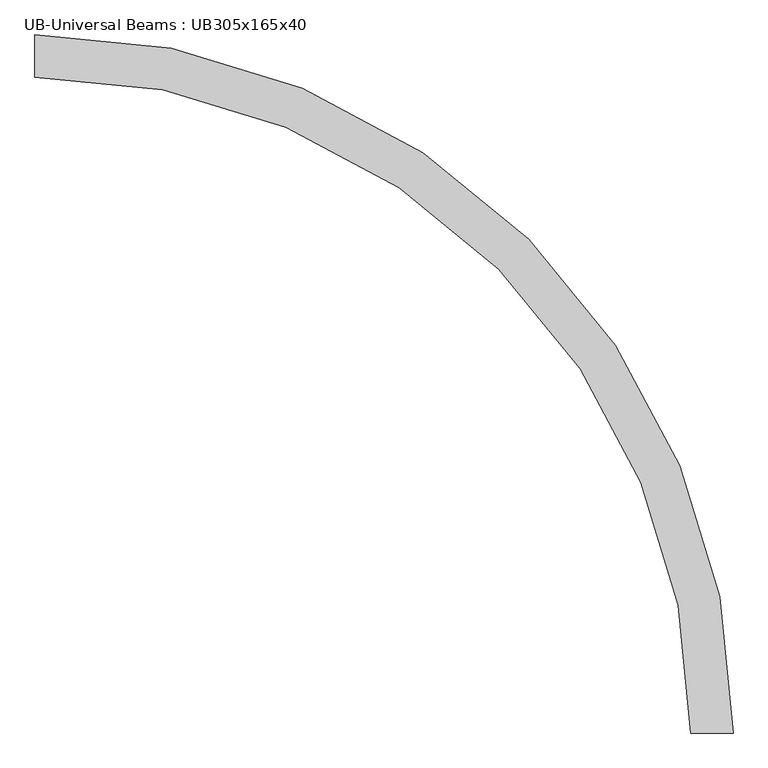
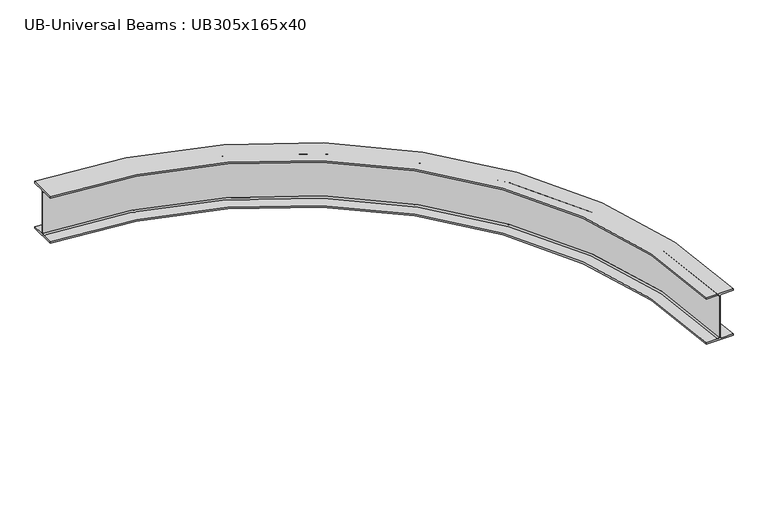
"""IFC4 building model written with IfcOpenShell, lengths in millimetres: beam geometry, UB-Universal Beams : UB305x165x40."""

from ifc_helpers import new_model, si_unit, point, frame, origin, place, context, project, spatial, polyline, circle_curve, ellipse_curve, trimmed, source, transform, mapped, element, save
from ifc_brep_helpers import plane_surface, cylinder_surface, revolved_surface, advanced_brep


def ub_universal_beams_ub305x165x40_a7bc032b(model_context):
    return source(origin(), model_context, "Body", "AdvancedBrep", [
        advanced_brep(
        [(2724.4689627, -2641.9689627, -141.5), (2653.8689627, -2641.9689627, -141.5), (2644.9689627, -2641.9689627, -132.6), (2644.9689627, -2641.9689627, 132.6), (2653.8689627, -2641.9689627, 141.5), (2724.4689627, -2641.9689627, 141.5), (2724.4689627, -2641.9689627, 151.7), (2559.4689627, -2641.9689627, 151.7), (2559.4689627, -2641.9689627, 141.5), (2630.0689627, -2641.9689627, 141.5), (2638.9689627, -2641.9689627, 132.6), (2638.9689627, -2641.9689627, -132.6), (2630.0689627, -2641.9689627, -141.5), (2559.4689627, -2641.9689627, -141.5), (2559.4689627, -2641.9689627, -151.7), (2724.4689627, -2641.9689627, -151.7), (0.0, 82.5, -141.5), (0.0, 82.5, -151.7), (0.0, -82.5, -151.7), (0.0, -82.5, -141.5), (0.0, -11.9, -141.5), (0.0, -3.0, -132.6), (0.0, -3.0, 132.6), (0.0, -11.9, 141.5), (0.0, -82.5, 141.5), (0.0, -82.5, 151.7), (0.0, 82.5, 151.7), (0.0, 82.5, 141.5), (0.0, 11.9, 141.5), (0.0, 3.0, 132.6), (0.0, 3.0, -132.6), (0.0, 11.9, -141.5)],
        [
            (0, 1),
            (1, 2, circle_curve(frame((2653.8689627, -2641.9689627, -132.6), z_axis=(0.0, 1.0, 0.0), x_axis=(-1.0, 0.0, 0.0)), 8.9)),
            (2, 3),
            (3, 4, circle_curve(frame((2653.8689627, -2641.9689627, 132.6), z_axis=(0.0, 1.0, 0.0), x_axis=(-1.0, 0.0, 0.0)), 8.9)),
            (4, 5),
            (5, 6),
            (6, 7),
            (7, 8),
            (8, 9),
            (9, 10, circle_curve(frame((2630.0689627, -2641.9689627, 132.6), z_axis=(0.0, 1.0, 0.0), x_axis=(-1.0, 0.0, 0.0)), 8.9)),
            (10, 11),
            (11, 12, circle_curve(frame((2630.0689627, -2641.9689627, -132.6), z_axis=(0.0, 1.0, 0.0), x_axis=(-1.0, 0.0, 0.0)), 8.9)),
            (12, 13),
            (13, 14),
            (14, 15),
            (15, 0),
            (16, 17),
            (17, 18),
            (18, 19),
            (19, 20),
            (20, 21, circle_curve(frame((0.0, -11.9, -132.6), z_axis=(1.0, 0.0, 0.0), x_axis=(0.0, -1.0, 0.0)), 8.9)),
            (21, 22),
            (22, 23, circle_curve(frame((0.0, -11.9, 132.6), z_axis=(1.0, 0.0, 0.0), x_axis=(0.0, -1.0, 0.0)), 8.9)),
            (23, 24),
            (24, 25),
            (25, 26),
            (26, 27),
            (27, 28),
            (28, 29, circle_curve(frame((0.0, 11.9, 132.6), z_axis=(1.0, 0.0, 0.0), x_axis=(0.0, -1.0, 0.0)), 8.9)),
            (29, 30),
            (30, 31, circle_curve(frame((0.0, 11.9, -132.6), z_axis=(1.0, 0.0, 0.0), x_axis=(0.0, -1.0, 0.0)), 8.9)),
            (31, 16),
            (0, 16, circle_curve(frame((0.0, -2641.9689627, -141.5), z_axis=(0.0, 0.0, 1.0), x_axis=(0.0, 1.0, 0.0)), 2724.4689627)),
            (31, 1, circle_curve(frame((0.0, -2641.9689627, -141.5), z_axis=(0.0, 0.0, -1.0), x_axis=(0.0, 1.0, 0.0)), 2653.8689627)),
            (30, 2, circle_curve(frame((0.0, -2641.9689627, -132.6), z_axis=(0.0, 0.0, -1.0), x_axis=(0.0, 1.0, 0.0)), 2644.9689627)),
            (29, 3, circle_curve(frame((0.0, -2641.9689627, 132.6), z_axis=(0.0, 0.0, -1.0), x_axis=(0.0, 1.0, 0.0)), 2644.9689627)),
            (28, 4, circle_curve(frame((0.0, -2641.9689627, 141.5), z_axis=(0.0, 0.0, -1.0), x_axis=(0.0, 1.0, 0.0)), 2653.8689627)),
            (27, 5, circle_curve(frame((0.0, -2641.9689627, 141.5), z_axis=(0.0, 0.0, -1.0), x_axis=(0.0, 1.0, 0.0)), 2724.4689627)),
            (26, 6, circle_curve(frame((0.0, -2641.9689627, 151.7), z_axis=(0.0, 0.0, -1.0), x_axis=(0.0, 1.0, 0.0)), 2724.4689627)),
            (25, 7, circle_curve(frame((0.0, -2641.9689627, 151.7), z_axis=(0.0, 0.0, -1.0), x_axis=(0.0, 1.0, 0.0)), 2559.4689627)),
            (24, 8, circle_curve(frame((0.0, -2641.9689627, 141.5), z_axis=(0.0, 0.0, -1.0), x_axis=(0.0, 1.0, 0.0)), 2559.4689627)),
            (23, 9, circle_curve(frame((0.0, -2641.9689627, 141.5), z_axis=(0.0, 0.0, -1.0), x_axis=(0.0, 1.0, 0.0)), 2630.0689627)),
            (22, 10, circle_curve(frame((0.0, -2641.9689627, 132.6), z_axis=(0.0, 0.0, -1.0), x_axis=(0.0, 1.0, 0.0)), 2638.9689627)),
            (21, 11, circle_curve(frame((0.0, -2641.9689627, -132.6), z_axis=(0.0, 0.0, -1.0), x_axis=(0.0, 1.0, 0.0)), 2638.9689627)),
            (20, 12, circle_curve(frame((0.0, -2641.9689627, -141.5), z_axis=(0.0, 0.0, -1.0), x_axis=(0.0, 1.0, 0.0)), 2630.0689627)),
            (19, 13, circle_curve(frame((0.0, -2641.9689627, -141.5), z_axis=(0.0, 0.0, -1.0), x_axis=(0.0, 1.0, 0.0)), 2559.4689627)),
            (18, 14, circle_curve(frame((0.0, -2641.9689627, -151.7), z_axis=(0.0, 0.0, -1.0), x_axis=(0.0, 1.0, 0.0)), 2559.4689627)),
            (17, 15, circle_curve(frame((0.0, -2641.9689627, -151.7), z_axis=(0.0, 0.0, -1.0), x_axis=(0.0, 1.0, 0.0)), 2724.4689627)),
        ],
        [
            plane_surface(frame((2641.9689627, -2641.9689627, 0.0), z_axis=(0.0, -1.0, 0.0), x_axis=(0.0, 0.0, 1.0))),
            plane_surface(frame((0.0, 0.0, 0.0), z_axis=(-1.0, 0.0, 0.0), x_axis=(0.0, 0.0, 1.0))),
            plane_surface(frame((0.0, -2641.9689627, -141.5), z_axis=(0.0, 0.0, 1.0), x_axis=(0.0, 1.0, 0.0))),
            revolved_surface(trimmed(ellipse_curve(frame((0.0, 11.9, -132.6), z_axis=(1.0, 0.0, 0.0), x_axis=(0.0, -1.0, 0.0)), 8.9, 8.9), [point((0.0, 3.0, -132.6))], [point((0.0, 11.9, -141.5))], True, "CARTESIAN"), (0.0, -2641.9689627, 0.0), (0.0, 0.0, -1.0)),
            cylinder_surface(frame((0.0, -2641.9689627, 0.0), z_axis=(0.0, 0.0, -1.0), x_axis=(0.0, 1.0, 0.0)), 2644.9689627),
            revolved_surface(trimmed(ellipse_curve(frame((0.0, 11.9, 132.6), z_axis=(1.0, 0.0, 0.0), x_axis=(0.0, -1.0, 0.0)), 8.9, 8.9), [point((0.0, 11.9, 141.5))], [point((0.0, 3.0, 132.6))], True, "CARTESIAN"), (0.0, -2641.9689627, 0.0), (0.0, 0.0, -1.0)),
            plane_surface(frame((0.0, -2641.9689627, 141.5), z_axis=(0.0, 0.0, -1.0), x_axis=(0.0, 1.0, 0.0))),
            cylinder_surface(frame((0.0, -2641.9689627, 0.0), z_axis=(0.0, 0.0, -1.0), x_axis=(0.0, 1.0, 0.0)), 2724.4689627),
            plane_surface(frame((0.0, -2641.9689627, 151.7), z_axis=(0.0, 0.0, 1.0), x_axis=(0.0, 1.0, 0.0))),
            revolved_surface(polyline([(0.0, -82.5, 141.5), (0.0, -82.5, 151.7)]), (0.0, -2641.9689627, 0.0), (0.0, 0.0, -1.0)),
            revolved_surface(trimmed(ellipse_curve(frame((0.0, -11.9, 132.6), z_axis=(1.0, 0.0, 0.0), x_axis=(0.0, -1.0, 0.0)), 8.9, 8.9), [point((0.0, -3.0, 132.6))], [point((0.0, -11.9, 141.5))], True, "CARTESIAN"), (0.0, -2641.9689627, 0.0), (0.0, 0.0, -1.0)),
            revolved_surface(polyline([(0.0, -3.0, -132.6), (0.0, -3.0, 132.6)]), (0.0, -2641.9689627, 0.0), (0.0, 0.0, -1.0)),
            revolved_surface(trimmed(ellipse_curve(frame((0.0, -11.9, -132.6), z_axis=(1.0, 0.0, 0.0), x_axis=(0.0, -1.0, 0.0)), 8.9, 8.9), [point((0.0, -11.9, -141.5))], [point((0.0, -3.0, -132.6))], True, "CARTESIAN"), (0.0, -2641.9689627, 0.0), (0.0, 0.0, -1.0)),
            revolved_surface(polyline([(0.0, -82.5, -151.7), (0.0, -82.5, -141.5)]), (0.0, -2641.9689627, 0.0), (0.0, 0.0, -1.0)),
            plane_surface(frame((0.0, -2641.9689627, -151.7), z_axis=(0.0, 0.0, -1.0), x_axis=(0.0, 1.0, 0.0))),
        ],
        [
            (0, [[1, 2, 3, 4, 5, 6, 7, 8, 9, 10, 11, 12, 13, 14, 15, 16]]),
            (1, [[17, 18, 19, 20, 21, 22, 23, 24, 25, 26, 27, 28, 29, 30, 31, 32]]),
            (2, [[-1, 33, -32, 34]]),
            (3, [[-2, -34, -31, 35]]),
            (4, [[-3, -35, -30, 36]]),
            (5, [[-4, -36, -29, 37]]),
            (6, [[-5, -37, -28, 38]]),
            (7, [[-6, -38, -27, 39]]),
            (8, [[-7, -39, -26, 40]]),
            (9, [[-8, -40, -25, 41]]),
            (6, [[-9, -41, -24, 42]]),
            (10, [[-10, -42, -23, 43]]),
            (11, [[-11, -43, -22, 44]]),
            (12, [[-12, -44, -21, 45]]),
            (2, [[-13, -45, -20, 46]]),
            (13, [[-14, -46, -19, 47]]),
            (14, [[-15, -47, -18, 48]]),
            (7, [[-16, -48, -17, -33]]),
        ],
    ),
    ])


if __name__ == "__main__":
    model = new_model("IFC4")
    model_context = context("Model", 3, world=origin())
    ifc_project = project(units=[si_unit("LENGTHUNIT", "METRE", prefix="MILLI")], contexts=[model_context])
    site = spatial("IfcSite", under=ifc_project)
    building = spatial("IfcBuilding", under=site)
    placement = place(None, origin())
    ub_universal_beams_ub305x165x40_shape = ub_universal_beams_ub305x165x40_a7bc032b(model_context)
    element("IfcBeam", 1, ObjectType="UB-Universal Beams : UB305x165x40", at=placement, inside=building, context=model_context, shape_type="MappedRepresentation", body=[
        mapped(ub_universal_beams_ub305x165x40_shape, transform((0.0, 0.0, 0.0), x_axis=(1.0, 0.0, 0.0), y_axis=(0.0, 1.0, 0.0), z_axis=(0.0, 0.0, 1.0))),
    ])
    save(model, "model.ifc")

# Revit data of these elements
# Type "UB-Universal Beams : UB305x165x40"
#   Section Name Key = "UB305X165X40"
#   Width = 16.5 cm
#   Web Thickness = 0.6 cm
#   Web Fillet = 0.89 cm
#   Warping Constant = 164000.0 cm⁶
#   Torsional Moment of Inertia = 14.70 cm⁴
#   Section Area = 51.3 cm²
#   Plastic Modulus weak axis = 142.0 cm³
#   Plastic Modulus strong axis = 623.0 cm³
#   Nominal Weight = 40.2999 kgf/m
#   Moment of Inertia weak axis = 764.00 cm⁴
#   Moment of Inertia strong axis = 8503.00 cm⁴
#   Height = 30.34 cm
#   Flange Thickness = 1.02 cm
#   Elastic Modulus weak axis = 92.6 cm³
#   Elastic Modulus strong axis = 560.0 cm³
#   Centroid Vertical = 15.17 cm
#   Centroid Horizontal = 8.25 cm
#   Bolt Spacing = 9.0 cm
#   Length [instance default] = 1500 mm
#   Structural Material [instance default] = Metal - Steel 43-275
#   Type Comments = ""
#   Assembly Code = ""
# Element 1 (IfcBeam, "UB-Universal Beams : UB305x165x40")
#   Materials on its faces: "Metal - Steel 43-275"
# Materials
#   "Metal - Steel 43-275": class "Metal", colour RGB 247 247 247, transparency 0, Cost = 0
